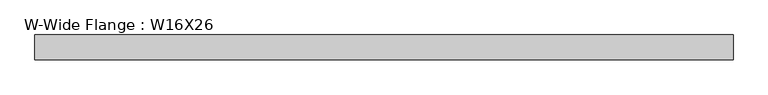
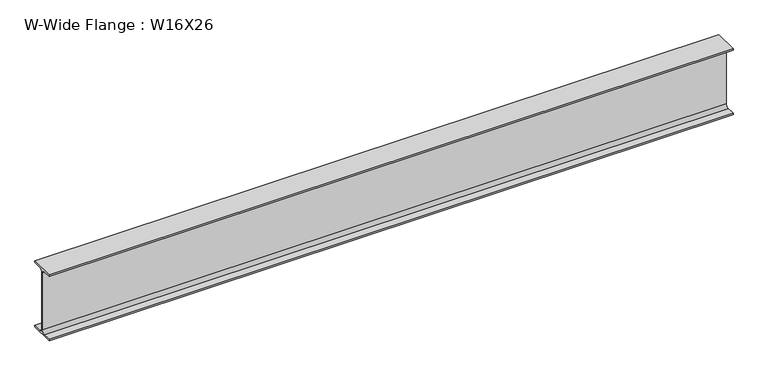
"""IFC4 building model written with IfcOpenShell, lengths in millimetres: beam geometry, W-Wide Flange : W16X26."""

from ifc_helpers import new_model, si_unit, point, frame, frame_2d, origin, place, context, project, spatial, polyline, circle_curve, trimmed, segment, composite_curve, outline, extrude, source, transform, mapped, element, save


def w_wide_flange_w16x26_d084e150(model_context):
    return source(origin(), model_context, "Body", "SweptSolid", [
        extrude(outline(composite_curve([segment(polyline([(69.85, -190.627), (69.85, -199.39), (-69.85, -199.39), (-69.85, -190.627), (-21.3995, -190.627)]), True, "CONTINUOUS"), segment(trimmed(circle_curve(frame_2d((-21.3995, -172.4025)), 18.2245), [point((-21.3995, -190.627))], [point((-3.175, -172.4025))], True, "CARTESIAN"), True, "CONTINUOUS"), segment(polyline([(-3.175, -172.4025), (-3.175, 172.4025)]), True, "CONTINUOUS"), segment(trimmed(circle_curve(frame_2d((-21.3995, 172.4025)), 18.2245), [point((-3.175, 172.4025))], [point((-21.3995, 190.627))], True, "CARTESIAN"), True, "CONTINUOUS"), segment(polyline([(-21.3995, 190.627), (-69.85, 190.627), (-69.85, 199.39), (69.85, 199.39), (69.85, 190.627), (21.3995, 190.627)]), True, "CONTINUOUS"), segment(trimmed(circle_curve(frame_2d((21.3995, 172.4025)), 18.2245), [point((21.3995, 190.627))], [point((3.175, 172.4025))], True, "CARTESIAN"), True, "CONTINUOUS"), segment(polyline([(3.175, 172.4025), (3.175, -172.4025)]), True, "CONTINUOUS"), segment(trimmed(circle_curve(frame_2d((21.3995, -172.4025)), 18.2245), [point((3.175, -172.4025))], [point((21.3995, -190.627))], True, "CARTESIAN"), True, "CONTINUOUS"), segment(polyline([(21.3995, -190.627), (69.85, -190.627)]), True, "CONTINUOUS")], self_intersect=False)), frame((-1955.8, 0.0, 0.0), z_axis=(1.0, 0.0, 0.0), x_axis=(0.0, 1.0, 0.0)), (0.0, 0.0, 1.0), 3911.6),
    ])


if __name__ == "__main__":
    model = new_model("IFC4")
    model_context = context("Model", 3, world=origin())
    ifc_project = project(units=[si_unit("LENGTHUNIT", "METRE", prefix="MILLI")], contexts=[model_context])
    site = spatial("IfcSite", under=ifc_project)
    building = spatial("IfcBuilding", under=site)
    placement = place(None, origin())
    w_wide_flange_w16x26_shape = w_wide_flange_w16x26_d084e150(model_context)
    element("IfcBeam", 1, ObjectType="W-Wide Flange : W16X26", at=placement, inside=building, context=model_context, shape_type="MappedRepresentation", body=[
        mapped(w_wide_flange_w16x26_shape, transform((0.0, 0.0, 0.0), x_axis=(1.0, 0.0, 0.0), y_axis=(0.0, 1.0, 0.0), z_axis=(0.0, 0.0, 1.0))),
    ])
    save(model, "model.ifc")

# Revit data of these elements
# Type "W-Wide Flange : W16X26"
#   Assembly Code = "B10"
#   W = 26
#   Length [instance default] = 5' - 0"
#   bf = 0' - 5 1/2"
#   d = 1' - 3.7"
#   k = 0' - 1 1/16"
#   k2 = 0' - 0.7175"
#   tf = 0' - 0.345"
#   tw = 0' - 0 1/4"
#   A = 0.0533333 SF
#   Structural Material [instance default] = Steel ASTM A992
# Element 1 (IfcBeam, "W-Wide Flange : W16X26")
#   Materials on its faces: "Steel ASTM A992"
# Materials
#   "Steel ASTM A992": class "Metal", colour RGB 199 199 199, transparency 0, Description = "Structural steel 50ksi", Cost = 0
